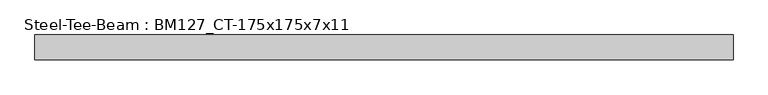
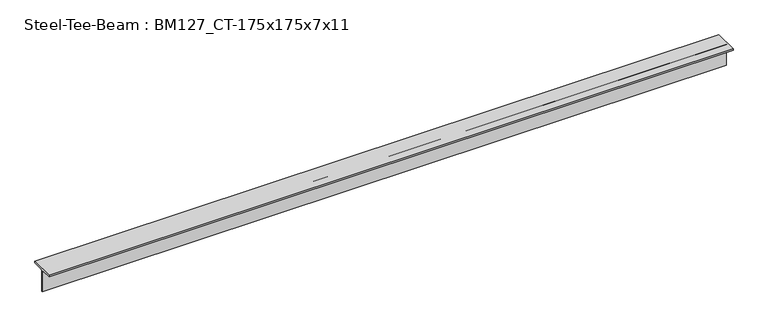
"""IFC4 building model written with IfcOpenShell, lengths in millimetres: beam geometry, Steel-Tee-Beam : BM127_CT-175x175x7x11."""

import ifcopenshell
import ifcopenshell.guid

model = None  # the IFC model being written
_history = None  # IfcOwnerHistory: only IFC2X3 demands one
_inside = {}  # id of a spatial element -> (the spatial element, [elements in it])
_under = {}  # id of a project, library or spatial element -> (it, [spatial elements below it])
_declared = {}  # id of a project -> (the project, [libraries it declares])
_typed = {}  # id of a type object -> (the type object, [elements of that type])
_made_of = {}  # id of a material, layer set ... -> (it, [elements and type objects made of it])


def new_model(schema):
    """Start an empty IFC model of exactly this schema.

    Asked for "IFC4X3", IfcOpenShell would pick the latest addendum, in which some entities
    have other attributes; the version numbers below select the first issue.
    IFC2X3 requires an IfcOwnerHistory on every rooted entity: one is made here for all.
    """
    global model, _history
    if schema == "IFC4X3":
        model = ifcopenshell.file(schema_version=(4, 3, 0, 0))
    else:
        model = ifcopenshell.file(schema=schema)
    _inside.clear()
    _under.clear()
    _declared.clear()
    _typed.clear()
    _made_of.clear()
    _history = None
    if model.schema == "IFC2X3":
        org = make("IfcOrganization", Name="unknown")
        user = make(
            "IfcPersonAndOrganization",
            ThePerson=make("IfcPerson", FamilyName="unknown"),
            TheOrganization=org,
        )
        app = make(
            "IfcApplication",
            ApplicationDeveloper=org,
            Version="unknown",
            ApplicationFullName="unknown",
            ApplicationIdentifier="unknown",
        )
        _history = make(
            "IfcOwnerHistory",
            OwningUser=user,
            OwningApplication=app,
            ChangeAction="ADDED",
            CreationDate=0,
        )
    return model


def make(cls, **values):
    """One entity of the class cls with the attributes given. An attribute that is None is left unset."""
    return model.create_entity(
        cls, **{name: value for name, value in values.items() if value is not None}
    )


def rooted(cls, **values):
    """An entity with a GlobalId (a new one), such as an element, a storey or a relation."""
    return make(cls, GlobalId=ifcopenshell.guid.new(), OwnerHistory=_history, **values)


def si_unit(unit_type, name, prefix=None):
    """IfcSIUnit, for example si_unit("LENGTHUNIT", "METRE", prefix="MILLI")."""
    return make("IfcSIUnit", UnitType=unit_type, Prefix=prefix, Name=name)


def assignment(units):
    """IfcUnitAssignment: the units of a project."""
    return None if units is None else make("IfcUnitAssignment", Units=units)


def point(xyz):
    """IfcCartesianPoint."""
    return None if xyz is None else make("IfcCartesianPoint", Coordinates=xyz)


def direction(xyz):
    """IfcDirection."""
    return None if xyz is None else make("IfcDirection", DirectionRatios=xyz)


def frame(location, z_axis=None, x_axis=None):
    """IfcAxis2Placement3D, a coordinate frame: its origin and axes. An axis left out is left unset."""
    return make(
        "IfcAxis2Placement3D",
        Location=point(location),
        Axis=direction(z_axis),
        RefDirection=direction(x_axis),
    )


def frame_2d(location, x_axis=None):
    """IfcAxis2Placement2D, a coordinate frame in the plane: its origin and x axis."""
    return make(
        "IfcAxis2Placement2D", Location=point(location), RefDirection=direction(x_axis)
    )


def origin():
    """The frame at (0, 0, 0) with its axes left unset."""
    return frame((0.0, 0.0, 0.0))


def place(relative_to, where):
    """IfcLocalPlacement: puts the frame where relative to a parent placement (None: the world)."""
    return make(
        "IfcLocalPlacement", PlacementRelTo=relative_to, RelativePlacement=where
    )


def context(
    kind, dimensions, precision=None, world=None, true_north=None, identifier=None
):
    """IfcGeometricRepresentationContext, for example the 3D "Model" context."""
    return make(
        "IfcGeometricRepresentationContext",
        ContextIdentifier=identifier,
        ContextType=kind,
        CoordinateSpaceDimension=dimensions,
        Precision=precision,
        WorldCoordinateSystem=world,
        TrueNorth=true_north,
    )


def project(units=None, contexts=None):
    """IfcProject with its units and contexts."""
    return rooted(
        "IfcProject",
        Name="project",
        RepresentationContexts=contexts,
        UnitsInContext=assignment(units),
    )


def spatial(cls, under=None, at=None, **own):
    """A site, building, storey or space (cls), placed at a placement, below another one or the project."""
    s = rooted(cls, ObjectPlacement=at, **own)
    if under is not None:
        _under.setdefault(under.id(), (under, []))[1].append(s)
    return s


def polyline(points):
    """IfcPolyline through the points."""
    return make("IfcPolyline", Points=[point(p) for p in points])


def circle_curve(where, radius):
    """IfcCircle in the frame where."""
    return make("IfcCircle", Position=where, Radius=radius)


def trimmed(basis, trim1, trim2, sense, master):
    """IfcTrimmedCurve: the piece of a basis curve between two trims."""
    return make(
        "IfcTrimmedCurve",
        BasisCurve=basis,
        Trim1=trim1,
        Trim2=trim2,
        SenseAgreement=sense,
        MasterRepresentation=master,
    )


def segment(curve, same_sense, transition):
    """IfcCompositeCurveSegment."""
    return make(
        "IfcCompositeCurveSegment",
        Transition=transition,
        SameSense=same_sense,
        ParentCurve=curve,
    )


def composite_curve(segments, self_intersect=None):
    """IfcCompositeCurve: segments joined end to end."""
    return make("IfcCompositeCurve", Segments=segments, SelfIntersect=self_intersect)


def outline(outer, holes=None, kind="AREA"):
    """IfcArbitraryClosedProfileDef: a profile drawn as a closed curve; with holes, ...WithVoids."""
    if holes is None:
        return make("IfcArbitraryClosedProfileDef", ProfileType=kind, OuterCurve=outer)
    return make(
        "IfcArbitraryProfileDefWithVoids",
        ProfileType=kind,
        OuterCurve=outer,
        InnerCurves=holes,
    )


def extrude(swept, where, along, depth):
    """IfcExtrudedAreaSolid: the profile swept, set in the frame where, extruded along a direction by depth."""
    return make(
        "IfcExtrudedAreaSolid",
        SweptArea=swept,
        Position=where,
        ExtrudedDirection=direction(along),
        Depth=depth,
    )


def shape(context_of_items, identifier, shape_type, items):
    """IfcShapeRepresentation: the items that make up one representation, for example the "Body"."""
    return make(
        "IfcShapeRepresentation",
        ContextOfItems=context_of_items,
        RepresentationIdentifier=identifier,
        RepresentationType=shape_type,
        Items=items,
    )


def source(mapping_origin, context_of_items, identifier, shape_type, items):
    """IfcRepresentationMap: a shape defined once, which mapped items show again and again."""
    return make(
        "IfcRepresentationMap",
        MappingOrigin=mapping_origin,
        MappedRepresentation=shape(context_of_items, identifier, shape_type, items),
    )


def transform(
    local_origin,
    x_axis=None,
    y_axis=None,
    z_axis=None,
    scale=None,
    scale2=None,
    scale3=None,
    uniform=True,
):
    """IfcCartesianTransformationOperator3D, or its non-uniform kind. x_axis, y_axis, z_axis: its Axis1, 2, 3."""
    if uniform:
        return make(
            "IfcCartesianTransformationOperator3D",
            Axis1=direction(x_axis),
            Axis2=direction(y_axis),
            LocalOrigin=point(local_origin),
            Scale=scale,
            Axis3=direction(z_axis),
        )
    return make(
        "IfcCartesianTransformationOperator3DnonUniform",
        Axis1=direction(x_axis),
        Axis2=direction(y_axis),
        LocalOrigin=point(local_origin),
        Scale=scale,
        Axis3=direction(z_axis),
        Scale2=scale2,
        Scale3=scale3,
    )


def mapped(mapping_source, mapping_target):
    """IfcMappedItem: shows the shape of a source again, moved by a transform."""
    return make(
        "IfcMappedItem", MappingSource=mapping_source, MappingTarget=mapping_target
    )


def made_of(thing, what):
    """Note that an element or type object is made of a material, layer set ...; save() writes the relation."""
    if what is not None:
        _made_of.setdefault(what.id(), (what, []))[1].append(thing)
    return thing


def element(
    cls,
    number,
    at=None,
    inside=None,
    cuts=None,
    type_object=None,
    material=None,
    context=None,
    identifier="Body",
    shape_type=None,
    held_by="IfcProductDefinitionShape",
    body=None,
    shapes=None,
    **own,
):
    """One element of the class cls, such as IfcWall. Its Tag is "e" and its number.

    at: its placement. inside: the storey or other place that contains it. cuts: it is an
    opening in that element (IfcRelVoidsElement). A single representation is given by context,
    identifier, shape_type and body (its items); several are given by shapes. held_by: the class
    of the entity that holds the representations. save() writes the other relations.
    """
    e = rooted(cls, Tag="e%d" % number, ObjectPlacement=at, **own)
    if body is not None:
        shapes = [shape(context, identifier, shape_type, body)]
    if shapes is not None:
        e.Representation = make(held_by, Representations=shapes)
    if inside is not None:
        _inside.setdefault(inside.id(), (inside, []))[1].append(e)
    if cuts is not None:
        rooted(
            "IfcRelVoidsElement", RelatingBuildingElement=cuts, RelatedOpeningElement=e
        )
    if type_object is not None:
        _typed.setdefault(type_object.id(), (type_object, []))[1].append(e)
    return made_of(e, material)


def aggregate(whole, parts):
    """IfcRelAggregates: a whole, such as a stair, and the parts it consists of."""
    return rooted("IfcRelAggregates", RelatingObject=whole, RelatedObjects=parts)


def save(model, path):
    """Write the relations noted so far, then the file.

    IfcRelAggregates (storeys below a building ...), IfcRelContainedInSpatialStructure (elements
    in a storey), IfcRelDefinesByType, IfcRelAssociatesMaterial and IfcRelDeclares: one each for
    every whole, place, type object, material and project.
    """
    for whole, parts in _under.values():
        aggregate(whole, parts)
    for where, things in _inside.values():
        rooted(
            "IfcRelContainedInSpatialStructure",
            RelatedElements=things,
            RelatingStructure=where,
        )
    for kind, things in _typed.values():
        rooted("IfcRelDefinesByType", RelatedObjects=things, RelatingType=kind)
    for what, things in _made_of.values():
        rooted("IfcRelAssociatesMaterial", RelatedObjects=things, RelatingMaterial=what)
    for by, libraries in _declared.values():
        rooted("IfcRelDeclares", RelatingContext=by, RelatedDefinitions=libraries)
    model.write(path)


def steel_tee_beam_bm127_ct_175x175x7x11_855b6dfc(model_context):
    return source(origin(), model_context, "Body", "SweptSolid", [
        extrude(outline(composite_curve([segment(polyline([(87.5, 87.5), (87.5, 76.5), (17.5, 76.5)]), True, "CONTINUOUS"), segment(trimmed(circle_curve(frame_2d((17.5, 62.5)), 14.0), [point((17.5, 76.5))], [point((3.5, 62.5))], True, "CARTESIAN"), True, "CONTINUOUS"), segment(polyline([(3.5, 62.5), (3.5, -87.5), (-3.5, -87.5), (-3.5, 62.5)]), True, "CONTINUOUS"), segment(trimmed(circle_curve(frame_2d((-17.5, 62.5)), 14.0), [point((-3.5, 62.5))], [point((-17.5, 76.5))], True, "CARTESIAN"), True, "CONTINUOUS"), segment(polyline([(-17.5, 76.5), (-87.5, 76.5), (-87.5, 87.5), (87.5, 87.5)]), True, "CONTINUOUS")], self_intersect=False)), frame((-2504.4959573, 0.0, 0.0), z_axis=(1.0, 0.0, 0.0), x_axis=(0.0, 1.0, 0.0)), (0.0, 0.0, 1.0), 4880.2539286),
    ])


if __name__ == "__main__":
    model = new_model("IFC4")
    model_context = context("Model", 3, world=origin())
    ifc_project = project(units=[si_unit("LENGTHUNIT", "METRE", prefix="MILLI")], contexts=[model_context])
    site = spatial("IfcSite", under=ifc_project)
    building = spatial("IfcBuilding", under=site)
    placement = place(None, origin())
    steel_tee_beam_bm127_ct_175x175x7x11_shape = steel_tee_beam_bm127_ct_175x175x7x11_855b6dfc(model_context)
    element("IfcBeam", 1, ObjectType="Steel-Tee-Beam : BM127_CT-175x175x7x11", at=placement, inside=building, context=model_context, shape_type="MappedRepresentation", body=[
        mapped(steel_tee_beam_bm127_ct_175x175x7x11_shape, transform((0.0, 0.0, 0.0), x_axis=(1.0, 0.0, 0.0), y_axis=(0.0, 1.0, 0.0), z_axis=(0.0, 0.0, 1.0))),
    ])
    save(model, "model.ifc")

# Revit data of these elements
# Type "Steel-Tee-Beam : BM127_CT-175x175x7x11"
#   Surface Area = 0.00 m²/m
#   Section Area = 31.57 cm²
#   Mass per Unit Length = 24.80 kg/m
#   Length [instance default] = 1524 mm
#   bf = 175 mm
#   d = 175 mm
#   k = 25 mm
#   kr = 14 mm
#   tf = 11 mm
#   tw = 7 mm
#   hec_material4 [instance default] = none
#   hec_material3 [instance default] = none
#   hec_material2 [instance default] = none
#   hec_material1 [instance default] = none
#   Structural Material [instance default] = Steel, 45-345
#   Assembly Code = ""
# Element 1 (IfcBeam, "Steel-Tee-Beam : BM127_CT-175x175x7x11")
#   hec_material3 = F01AC000-00002_Building/Shelter Fire Proofing Work_Intumescent Coating Type_1 hr. rating (UL 1709))
#   hec_material2 = S01AA010-00002_Main Steel Structure Fabrication Work_Shelter/Building_Steel Painting/Coating_for Fireproofed Steel Surface, Surface Preparation & Primer Coat
#   hec_material1 = S03AA029-00001_Main Steel Structure Erection Work_Shelter/Building_Light Steel
#   Structural Material = S01AA003-00001_Main Steel Structure Fabrication Work_Shelter/Building_Light Steel - Standard
#   Materials on its faces: "S01AA003-00001_Main Steel Structure Fabrication Work_Shelter/Building_Light Steel - Standard"
# Materials
#   "Steel, 45-345": class "Metal", colour RGB 189 187 185, transparency 0, Description = "Steel 345 MPa", Cost = 0
#   "S01AA003-00001_Main Steel Structure Fabrication Work_Shelter/Building_Light Steel - Standard": class "Metal", colour RGB 120 120 120, transparency 0, Comments = "(30KG/M>Weight)", Description = "Structural steel 50ksi", W00) Work Master Code = "S01AA003-00001", W01) Work Master_Lv1 = "Main Steel Structure Fabrication Work", W02) Work Master_Lv2 = "Shelter/Building", W03) Work Master_Spec.1 = "Light Steel - Standard (30KG/M>Weight)", Cost = 0
#   "F01AC000-00002_Building/Shelter Fire Proofing Work_Intumescent Coating Type_1 hr. rating (UL 1709))": class "Metal", colour RGB 255 128 128, transparency 0, Description = "Paint finished steel", W00) Work Master Code = "F01AC000-00002", W01) Work Master_Lv1 = "Building/Shelter Fire Proofing Work", W02) Work Master_Lv2 = "Intumescent Coating Type", W03) Work Master_Spec.1 = "1 hr. rating (UL 1709)", Cost = 0
#   "S01AA010-00002_Main Steel Structure Fabrication Work_Shelter/Building_Steel Painting/Coating_for Fireproofed Steel Surface, Surface Preparation & Primer Coat": class "Metal", colour RGB 120 120 120, transparency 0, Description = "Paint finished steel", W00) Work Master Code = "SS01AA010-00002", W01) Work Master_Lv1 = "Main Steel Structure Fabrication Work", W02) Work Master_Lv2 = "Shelter/Building", W03) Work Master_Spec.1 = "Steel Painting/Coating", W04) Work Master_Spec.2 = "for Fireproofed Steel Surface, Surface Preparation & Primer Coat", Cost = 0
#   "S03AA029-00001_Main Steel Structure Erection Work_Shelter/Building_Light Steel": class "Metal", colour RGB 120 120 120, transparency 0, Comments = "(30KG/M>Weight)", Description = "Structural steel 50ksi", W00) Work Master Code = "S03AA029-00001", W01) Work Master_Lv1 = "Main Steel Structure Erection Work", W02) Work Master_Lv2 = "Shelter/Building", W03) Work Master_Spec.1 = "Light Steel (30KG/M>Weight)", Cost = 0
